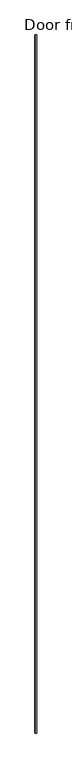
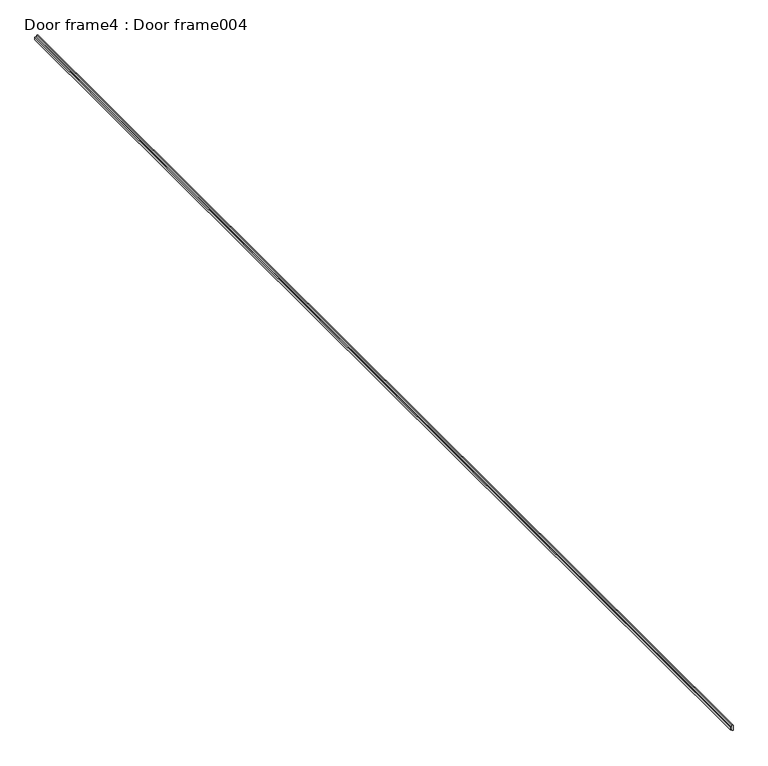
"""IFC4 building model written with IfcOpenShell, lengths in millimetres: proxy geometry, Door frame4 : Door frame004."""

from ifc_helpers import new_model, si_unit, frame, origin, place, context, project, spatial, polyline, outline, extrude, source, transform, mapped, element, save


def door_frame4_door_frame004_03d84ab6(model_context):
    return source(origin(), model_context, "Body", "SweptSolid", [
        extrude(outline(polyline([(36685.3750947, 15525.9592515), (36685.3750947, 15524.8924515), (36680.8030947, 15524.8924515), (36680.8030947, 15525.9592515), (36682.2000947, 15525.9592515), (36682.2000947, 15527.7372515), (36678.7014343, 15527.7372515), (36678.7014343, 15529.9292246), (36687.4772673, 15529.9292246), (36687.4772673, 15527.7373022), (36683.9780947, 15527.7373022), (36683.9780947, 15525.9592515), (36685.3750947, 15525.9592515)])), frame((0.0, -1052.8906567, 0.0), z_axis=(0.0, 1.0, 0.0), x_axis=(0.0, 0.0, 1.0)), (0.0, 0.0, 1.0), 1999.85),
    ])


if __name__ == "__main__":
    model = new_model("IFC4")
    model_context = context("Model", 3, world=origin())
    ifc_project = project(units=[si_unit("LENGTHUNIT", "METRE", prefix="MILLI")], contexts=[model_context])
    site = spatial("IfcSite", under=ifc_project)
    building = spatial("IfcBuilding", under=site)
    placement = place(None, origin())
    door_frame4_door_frame004_shape = door_frame4_door_frame004_03d84ab6(model_context)
    element("IfcBuildingElementProxy", 1, Name="Door frame4 : Door frame004", ObjectType="Door frame4 : Door frame004", at=placement, inside=building, context=model_context, shape_type="MappedRepresentation", body=[
        mapped(door_frame4_door_frame004_shape, transform((0.0, 0.0, 0.0), x_axis=(1.0, 0.0, 0.0), y_axis=(0.0, 1.0, 0.0), z_axis=(0.0, 0.0, 1.0))),
    ])
    save(model, "model.ifc")

# Revit data of these elements
# Type "Door frame4 : Door frame004"
#   NameOverride = "Door frame004"
# Element 1 (IfcBuildingElementProxy, "Door frame4 : Door frame004")
#   Materials on its faces: "FLEETWOOD SERIES T-3200 SINGLE SWING DOOR FRAME"
# Materials
#   "FLEETWOOD SERIES T-3200 SINGLE SWING DOOR FRAME": class "Unassigned", colour RGB 128 128 128, transparency 0, Cost = 0
